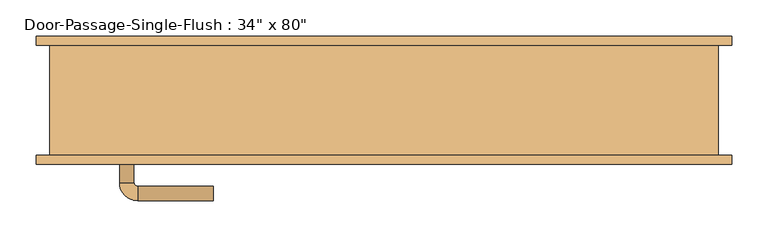
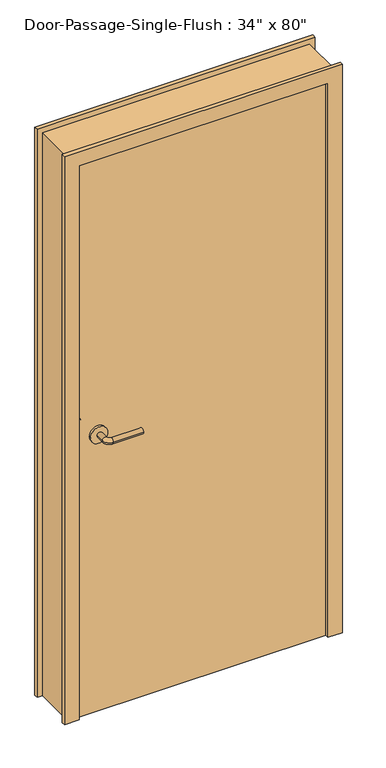
"""IFC4 building model written with IfcOpenShell, lengths in millimetres: door geometry."""

from ifc_helpers import new_model, si_unit, point, frame, frame_2d, origin, origin_with_axes, place, context, project, spatial, polyline, circle_curve, ellipse_curve, trimmed, segment, composite_curve, outline, extrude, faceted_brep, source, transform, mapped, element, save
from ifc_brep_helpers import plane_surface, cylinder_surface, revolved_surface, advanced_brep


def door_2354040f(model_context):
    return source(origin(), model_context, "Body", "SolidModel", [
        advanced_brep(
        [(-366.790625, -23.75, 1016.0), (-346.790625, -23.75, 1016.0), (-366.790625, 6.25, 1016.0), (-346.790625, 6.25, 1016.0), (-341.790625, 11.25, 1016.0), (-341.790625, 31.25, 1016.0), (-236.790625, 31.25, 1016.0), (-236.790625, 11.25, 1016.0)],
        [
            (0, 1, circle_curve(frame((-356.790625, -23.75, 1016.0), z_axis=(0.0, -1.0, 0.0), x_axis=(1.0, 0.0, 0.0)), 10.0)),
            (1, 0, circle_curve(frame((-356.790625, -23.75, 1016.0), z_axis=(0.0, -1.0, 0.0), x_axis=(1.0, 0.0, 0.0)), 10.0)),
            (0, 2),
            (2, 3, circle_curve(frame((-356.790625, 6.25, 1016.0), z_axis=(0.0, -1.0, 0.0), x_axis=(1.0, 0.0, 0.0)), 10.0)),
            (3, 1),
            (3, 2, circle_curve(frame((-356.790625, 6.25, 1016.0), z_axis=(0.0, -1.0, 0.0), x_axis=(1.0, 0.0, 0.0)), 10.0)),
            (4, 3, circle_curve(frame((-341.790625, 6.25, 1016.0), z_axis=(0.0, 0.0, 1.0), x_axis=(-1.0, 0.0, 0.0)), 5.0)),
            (2, 5, circle_curve(frame((-341.790625, 6.25, 1016.0), z_axis=(0.0, 0.0, -1.0), x_axis=(-1.0, 0.0, 0.0)), 25.0)),
            (5, 4, circle_curve(frame((-341.790625, 21.25, 1016.0), z_axis=(-1.0, 0.0, 0.0), x_axis=(0.0, -1.0, 0.0)), 10.0)),
            (4, 5, circle_curve(frame((-341.790625, 21.25, 1016.0), z_axis=(-1.0, 0.0, 0.0), x_axis=(0.0, -1.0, 0.0)), 10.0)),
            (6, 7, circle_curve(frame((-236.790625, 21.25, 1016.0), z_axis=(1.0, 0.0, 0.0), x_axis=(0.0, -1.0, 0.0)), 10.0)),
            (7, 6, circle_curve(frame((-236.790625, 21.25, 1016.0), z_axis=(1.0, 0.0, 0.0), x_axis=(0.0, -1.0, 0.0)), 10.0)),
            (5, 6),
            (7, 4),
        ],
        [
            plane_surface(frame((-356.790625, -23.75, 1016.0), z_axis=(0.0, -1.0, 0.0), x_axis=(0.0, 0.0, 1.0))),
            cylinder_surface(frame((-356.790625, -23.75, 1016.0), z_axis=(0.0, -1.0, 0.0), x_axis=(1.0, 0.0, 0.0)), 10.0),
            revolved_surface(trimmed(ellipse_curve(frame((-356.790625, 6.25, 1016.0), z_axis=(0.0, -1.0, 0.0), x_axis=(1.0, 0.0, 0.0)), 10.0, 10.0), [point((-366.790625, 6.25, 1016.0))], [point((-346.790625, 6.25, 1016.0))], True, "CARTESIAN"), (-341.790625, 6.25, 1016.0), (0.0, 0.0, -1.0)),
            revolved_surface(trimmed(ellipse_curve(frame((-356.790625, 6.25, 1016.0), z_axis=(0.0, -1.0, 0.0), x_axis=(1.0, 0.0, 0.0)), 10.0, 10.0), [point((-346.790625, 6.25, 1016.0))], [point((-366.790625, 6.25, 1016.0))], True, "CARTESIAN"), (-341.790625, 6.25, 1016.0), (0.0, 0.0, -1.0)),
            plane_surface(frame((-236.790625, 21.25, 1016.0), z_axis=(1.0, 0.0, 0.0), x_axis=(0.0, 0.0, 1.0))),
            cylinder_surface(frame((-341.790625, 21.25, 1016.0), z_axis=(-1.0, 0.0, 0.0), x_axis=(0.0, -1.0, 0.0)), 10.0),
        ],
        [
            (0, [[1, 2]]),
            (1, [[-1, 3, 4, 5]]),
            (1, [[-2, -5, 6, -3]]),
            (2, [[7, -4, 8, 9]]),
            (3, [[-8, -6, -7, 10]]),
            (4, [[11, 12]]),
            (5, [[-9, 13, -12, 14]]),
            (5, [[-10, -14, -11, -13]]),
        ],
    ),
        extrude(outline(composite_curve([segment(trimmed(circle_curve(frame_2d((1016.0, -359.290625)), 30.0), [point((1016.0, -389.290625))], [point((1016.0, -329.290625))], False, "CARTESIAN"), True, "CONTINUOUS"), segment(trimmed(circle_curve(frame_2d((1016.0, -359.290625)), 30.0), [point((1016.0, -329.290625))], [point((1016.0, -389.290625))], False, "CARTESIAN"), True, "CONTINUOUS")], self_intersect=False)), frame((0.0, -31.75, 0.0), z_axis=(0.0, 1.0, 0.0), x_axis=(0.0, 0.0, 1.0)), (0.0, 0.0, 1.0), 8.0),
        advanced_brep(
        [(-366.790625, -90.55, 1016.0), (-346.790625, -90.55, 1016.0), (-346.790625, -120.55, 1016.0), (-366.790625, -120.55, 1016.0), (-341.790625, -125.55, 1016.0), (-341.790625, -145.55, 1016.0), (-236.790625, -145.55, 1016.0), (-236.790625, -125.55, 1016.0)],
        [
            (0, 1, circle_curve(frame((-356.790625, -90.55, 1016.0), z_axis=(0.0, 1.0, 0.0), x_axis=(1.0, 0.0, 0.0)), 10.0)),
            (1, 0, circle_curve(frame((-356.790625, -90.55, 1016.0), z_axis=(0.0, 1.0, 0.0), x_axis=(1.0, 0.0, 0.0)), 10.0)),
            (1, 2),
            (2, 3, circle_curve(frame((-356.790625, -120.55, 1016.0), z_axis=(0.0, 1.0, 0.0), x_axis=(1.0, 0.0, 0.0)), 10.0)),
            (3, 0),
            (3, 2, circle_curve(frame((-356.790625, -120.55, 1016.0), z_axis=(0.0, 1.0, 0.0), x_axis=(1.0, 0.0, 0.0)), 10.0)),
            (4, 5, circle_curve(frame((-341.790625, -135.55, 1016.0), z_axis=(-1.0, 0.0, 0.0), x_axis=(0.0, 1.0, 0.0)), 10.0)),
            (5, 3, circle_curve(frame((-341.790625, -120.55, 1016.0), z_axis=(0.0, 0.0, -1.0), x_axis=(-1.0, 0.0, 0.0)), 25.0)),
            (2, 4, circle_curve(frame((-341.790625, -120.55, 1016.0), z_axis=(0.0, 0.0, 1.0), x_axis=(-1.0, 0.0, 0.0)), 5.0)),
            (5, 4, circle_curve(frame((-341.790625, -135.55, 1016.0), z_axis=(-1.0, 0.0, 0.0), x_axis=(0.0, 1.0, 0.0)), 10.0)),
            (6, 7, circle_curve(frame((-236.790625, -135.55, 1016.0), z_axis=(1.0, 0.0, 0.0), x_axis=(0.0, 1.0, 0.0)), 10.0)),
            (7, 6, circle_curve(frame((-236.790625, -135.55, 1016.0), z_axis=(1.0, 0.0, 0.0), x_axis=(0.0, 1.0, 0.0)), 10.0)),
            (4, 7),
            (6, 5),
        ],
        [
            plane_surface(frame((-356.790625, -90.55, 1016.0), z_axis=(0.0, 1.0, 0.0), x_axis=(0.0, 0.0, 1.0))),
            cylinder_surface(frame((-356.790625, -90.55, 1016.0), z_axis=(0.0, 1.0, 0.0), x_axis=(1.0, 0.0, 0.0)), 10.0),
            revolved_surface(trimmed(ellipse_curve(frame((-356.790625, -120.55, 1016.0), z_axis=(0.0, -1.0, 0.0), x_axis=(1.0, 0.0, 0.0)), 10.0, 10.0), [point((-366.790625, -120.55, 1016.0))], [point((-346.790625, -120.55, 1016.0))], True, "CARTESIAN"), (-341.790625, -120.55, 1016.0), (0.0, 0.0, -1.0)),
            revolved_surface(trimmed(ellipse_curve(frame((-356.790625, -120.55, 1016.0), z_axis=(0.0, -1.0, 0.0), x_axis=(1.0, 0.0, 0.0)), 10.0, 10.0), [point((-346.790625, -120.55, 1016.0))], [point((-366.790625, -120.55, 1016.0))], True, "CARTESIAN"), (-341.790625, -120.55, 1016.0), (0.0, 0.0, -1.0)),
            plane_surface(frame((-236.790625, -135.55, 1016.0), z_axis=(1.0, 0.0, 0.0), x_axis=(0.0, 0.0, 1.0))),
            cylinder_surface(frame((-341.790625, -135.55, 1016.0), z_axis=(-1.0, 0.0, 0.0), x_axis=(0.0, 1.0, 0.0)), 10.0),
        ],
        [
            (0, [[1, 2]]),
            (1, [[3, 4, 5, -2]]),
            (1, [[-5, 6, -3, -1]]),
            (2, [[7, 8, -4, 9]]),
            (3, [[10, -9, -6, -8]]),
            (4, [[11, 12]]),
            (5, [[13, -11, 14, -7]]),
            (5, [[-14, -12, -13, -10]]),
        ],
    ),
        extrude(outline(composite_curve([segment(trimmed(circle_curve(frame_2d((1016.0, -359.290625)), 30.0), [point((1016.0, -389.290625))], [point((1016.0, -329.290625))], False, "CARTESIAN"), True, "CONTINUOUS"), segment(trimmed(circle_curve(frame_2d((1016.0, -359.290625)), 30.0), [point((1016.0, -329.290625))], [point((1016.0, -389.290625))], False, "CARTESIAN"), True, "CONTINUOUS")], self_intersect=False)), frame((0.0, -90.55, 0.0), z_axis=(0.0, 1.0, 0.0), x_axis=(0.0, 0.0, 1.0)), (0.0, 0.0, 1.0), 8.0),
        faceted_brep([(431.8, -95.25, 0.0), (431.8, -26.9875, 0.0), (415.925, -26.9875, 0.0), (415.925, 11.1125, 0.0), (431.8, 11.1125, 0.0), (431.8, 82.55, 0.0), (482.6, 82.55, 0.0), (482.6, 69.85, 0.0), (463.55, 69.85, 0.0), (463.55, -82.55, 0.0), (482.6, -82.55, 0.0), (482.6, -95.25, 0.0), (482.6, -95.25, 2082.8), (-482.6, -95.25, 2082.8), (-482.6, -95.25, 0.0), (-431.8, -95.25, 0.0), (-431.8, -95.25, 2032.0), (431.8, -95.25, 2032.0), (482.6, -82.55, 2082.8), (463.55, -82.55, 2063.75), (-463.55, -82.55, 2063.75), (-463.55, -82.55, 0.0), (-482.6, -82.55, 0.0), (-482.6, -82.55, 2082.8), (463.55, 69.85, 2063.75), (482.6, 69.85, 2082.8), (-482.6, 69.85, 2082.8), (-482.6, 69.85, 0.0), (-463.55, 69.85, 0.0), (-463.55, 69.85, 2063.75), (482.6, 82.55, 2082.8), (431.8, 82.55, 2032.0), (-431.8, 82.55, 2032.0), (-431.8, 82.55, 0.0), (-482.6, 82.55, 0.0), (-482.6, 82.55, 2082.8), (431.8, 11.1125, 2032.0), (415.925, 11.1125, 2016.125), (-415.925, 11.1125, 2016.125), (-415.925, 11.1125, 0.0), (-431.8, 11.1125, 0.0), (-431.8, 11.1125, 2032.0), (415.925, -26.9875, 2016.125), (431.8, -26.9875, 2032.0), (-431.8, -26.9875, 2032.0), (-431.8, -26.9875, 0.0), (-415.925, -26.9875, 0.0), (-415.925, -26.9875, 2016.125)], [[[0, 1, 2, 3, 4, 5, 6, 7, 8, 9, 10, 11]], [[11, 12, 13, 14, 15, 16, 17, 0]], [[10, 18, 12, 11]], [[9, 19, 20, 21, 22, 23, 18, 10]], [[8, 24, 19, 9]], [[7, 25, 26, 27, 28, 29, 24, 8]], [[6, 30, 25, 7]], [[5, 31, 32, 33, 34, 35, 30, 6]], [[4, 36, 31, 5]], [[3, 37, 38, 39, 40, 41, 36, 4]], [[2, 42, 37, 3]], [[1, 43, 44, 45, 46, 47, 42, 2]], [[0, 17, 43, 1]], [[18, 23, 13, 12]], [[24, 29, 20, 19]], [[30, 35, 26, 25]], [[36, 41, 32, 31]], [[42, 47, 38, 37]], [[17, 16, 44, 43]], [[15, 14, 22, 21, 28, 27, 34, 33, 40, 39, 46, 45]], [[23, 22, 14, 13]], [[29, 28, 21, 20]], [[35, 34, 27, 26]], [[41, 40, 33, 32]], [[47, 46, 39, 38]], [[16, 15, 45, 44]]]),
        extrude(outline(polyline([(431.8, -31.75), (431.8, -82.55), (-431.8, -82.55), (-431.8, -31.75), (431.8, -31.75)])), origin_with_axes(), (0.0, 0.0, 1.0), 2032.0),
    ])


if __name__ == "__main__":
    model = new_model("IFC4")
    model_context = context("Model", 3, world=origin())
    ifc_project = project(units=[si_unit("LENGTHUNIT", "METRE", prefix="MILLI")], contexts=[model_context])
    site = spatial("IfcSite", under=ifc_project)
    building = spatial("IfcBuilding", under=site)
    placement = place(None, origin())
    door_shape = door_2354040f(model_context)
    element("IfcDoor", 1, ObjectType="Door-Passage-Single-Flush : 34\" x 80\"", at=placement, inside=building, context=model_context, shape_type="MappedRepresentation", body=[
        mapped(door_shape, transform((0.0, 0.0, 0.0), x_axis=(1.0, 0.0, 0.0), y_axis=(0.0, 1.0, 0.0), z_axis=(0.0, 0.0, 1.0))),
    ])
    save(model, "model.ifc")

# Revit data of these elements
# Type "Door-Passage-Single-Flush : 34\" x 80\""
#   Type Mark = "14"
#   Assembly Code = "C1020"
#   Analytic Construction = "Wooden"
#   Thickness = 0' - 2"
#   Thermal Resistance (R) = 2.5876 (h·ft²·°F)/BTU
#   Swing Angle [instance default] = 90.00°
#   Strike Height = 3' - 4"
#   Rough Width [instance default] = 3' - 2"
#   Rough Height [instance default] = 7' - 0"
#   Masonry Inset [instance default] = 0' - 1"
#   Masonry Frame Depth = 0' - 5 3/4"
#   MF Opening Width [instance default] = 0' - 4"
#   MF Opening Height [instance default] = 0' - 4"
#   Inset Calculate [instance default] = 0' - 4"
#   Heat Transfer Coefficient (U) = 0.3865 BTU/(h·ft²·°F)
#   Height = 6' - 8"
#   Width = 2' - 10"
#   Masonry Frame [instance default] = yes
#   Dry Wall Frame [instance default] = no
#   Panel Material = Wood - Birch
#   Door Handle Material = Aluminum
#   Frame Material = Door - Frame
#   Visual Light Transmittance = 0
#   Solar Heat Gain Coefficient = 0
#   Function = (empty or 0)
#   Wall Closure = (empty or 0)
# Element 1 (IfcDoor, "Door-Passage-Single-Flush : 34\" x 80\"")
#   Rough Width = 3' - 0 1/2"
#   Rough Height = 6' - 9 1/4"
#   MF Opening Width = 0' - 2 1/2"
#   MF Opening Height = 0' - 1 1/4"
#   Inset Calculate = 0' - 3"
#   Masonry Frame = no
#   Dry Wall Frame = yes
#   Materials on its faces: "Door - Frame", "Aluminum", "Wood - Birch"
# Materials
#   "Wood - Birch": class "Unassigned", colour RGB 224 178 126, transparency 0
#   "Aluminum": class "Metal", colour RGB 244 244 244, transparency 0, Description = "Aluminum 6061", Cost = 0
#   "Door - Frame": class "Unassigned", colour RGB 118 70 51, transparency 0
